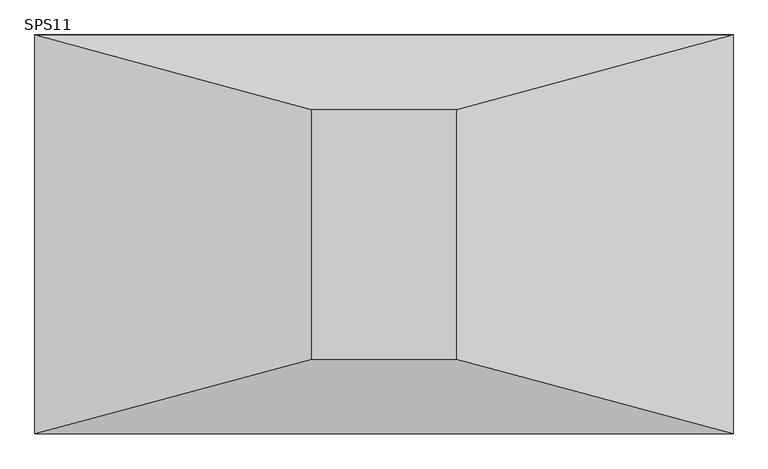
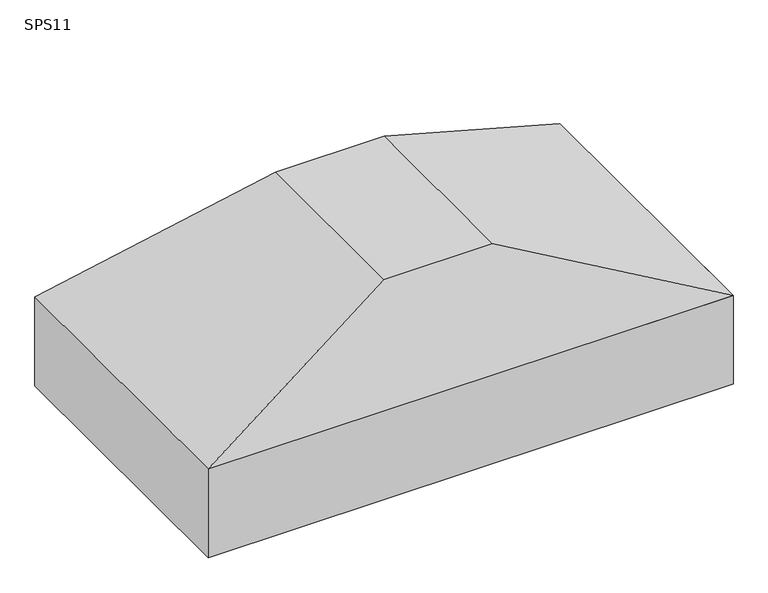
"""IFC4 building model written with IfcOpenShell, lengths in millimetres: fastener geometry, TQS - Sapata : SPS11."""

import ifcopenshell
import ifcopenshell.guid

model = None  # the IFC model being written
_history = None  # IfcOwnerHistory: only IFC2X3 demands one
_inside = {}  # id of a spatial element -> (the spatial element, [elements in it])
_under = {}  # id of a project, library or spatial element -> (it, [spatial elements below it])
_declared = {}  # id of a project -> (the project, [libraries it declares])
_typed = {}  # id of a type object -> (the type object, [elements of that type])
_made_of = {}  # id of a material, layer set ... -> (it, [elements and type objects made of it])


def new_model(schema):
    """Start an empty IFC model of exactly this schema.

    Asked for "IFC4X3", IfcOpenShell would pick the latest addendum, in which some entities
    have other attributes; the version numbers below select the first issue.
    IFC2X3 requires an IfcOwnerHistory on every rooted entity: one is made here for all.
    """
    global model, _history
    if schema == "IFC4X3":
        model = ifcopenshell.file(schema_version=(4, 3, 0, 0))
    else:
        model = ifcopenshell.file(schema=schema)
    _inside.clear()
    _under.clear()
    _declared.clear()
    _typed.clear()
    _made_of.clear()
    _history = None
    if model.schema == "IFC2X3":
        org = make("IfcOrganization", Name="unknown")
        user = make(
            "IfcPersonAndOrganization",
            ThePerson=make("IfcPerson", FamilyName="unknown"),
            TheOrganization=org,
        )
        app = make(
            "IfcApplication",
            ApplicationDeveloper=org,
            Version="unknown",
            ApplicationFullName="unknown",
            ApplicationIdentifier="unknown",
        )
        _history = make(
            "IfcOwnerHistory",
            OwningUser=user,
            OwningApplication=app,
            ChangeAction="ADDED",
            CreationDate=0,
        )
    return model


def make(cls, **values):
    """One entity of the class cls with the attributes given. An attribute that is None is left unset."""
    return model.create_entity(
        cls, **{name: value for name, value in values.items() if value is not None}
    )


def rooted(cls, **values):
    """An entity with a GlobalId (a new one), such as an element, a storey or a relation."""
    return make(cls, GlobalId=ifcopenshell.guid.new(), OwnerHistory=_history, **values)


def si_unit(unit_type, name, prefix=None):
    """IfcSIUnit, for example si_unit("LENGTHUNIT", "METRE", prefix="MILLI")."""
    return make("IfcSIUnit", UnitType=unit_type, Prefix=prefix, Name=name)


def assignment(units):
    """IfcUnitAssignment: the units of a project."""
    return None if units is None else make("IfcUnitAssignment", Units=units)


def point(xyz):
    """IfcCartesianPoint."""
    return None if xyz is None else make("IfcCartesianPoint", Coordinates=xyz)


def direction(xyz):
    """IfcDirection."""
    return None if xyz is None else make("IfcDirection", DirectionRatios=xyz)


def frame(location, z_axis=None, x_axis=None):
    """IfcAxis2Placement3D, a coordinate frame: its origin and axes. An axis left out is left unset."""
    return make(
        "IfcAxis2Placement3D",
        Location=point(location),
        Axis=direction(z_axis),
        RefDirection=direction(x_axis),
    )


def origin():
    """The frame at (0, 0, 0) with its axes left unset."""
    return frame((0.0, 0.0, 0.0))


def place(relative_to, where):
    """IfcLocalPlacement: puts the frame where relative to a parent placement (None: the world)."""
    return make(
        "IfcLocalPlacement", PlacementRelTo=relative_to, RelativePlacement=where
    )


def context(
    kind, dimensions, precision=None, world=None, true_north=None, identifier=None
):
    """IfcGeometricRepresentationContext, for example the 3D "Model" context."""
    return make(
        "IfcGeometricRepresentationContext",
        ContextIdentifier=identifier,
        ContextType=kind,
        CoordinateSpaceDimension=dimensions,
        Precision=precision,
        WorldCoordinateSystem=world,
        TrueNorth=true_north,
    )


def project(units=None, contexts=None):
    """IfcProject with its units and contexts."""
    return rooted(
        "IfcProject",
        Name="project",
        RepresentationContexts=contexts,
        UnitsInContext=assignment(units),
    )


def spatial(cls, under=None, at=None, **own):
    """A site, building, storey or space (cls), placed at a placement, below another one or the project."""
    s = rooted(cls, ObjectPlacement=at, **own)
    if under is not None:
        _under.setdefault(under.id(), (under, []))[1].append(s)
    return s


def polyline(points):
    """IfcPolyline through the points."""
    return make("IfcPolyline", Points=[point(p) for p in points])


def outline(outer, holes=None, kind="AREA"):
    """IfcArbitraryClosedProfileDef: a profile drawn as a closed curve; with holes, ...WithVoids."""
    if holes is None:
        return make("IfcArbitraryClosedProfileDef", ProfileType=kind, OuterCurve=outer)
    return make(
        "IfcArbitraryProfileDefWithVoids",
        ProfileType=kind,
        OuterCurve=outer,
        InnerCurves=holes,
    )


def extrude(swept, where, along, depth):
    """IfcExtrudedAreaSolid: the profile swept, set in the frame where, extruded along a direction by depth."""
    return make(
        "IfcExtrudedAreaSolid",
        SweptArea=swept,
        Position=where,
        ExtrudedDirection=direction(along),
        Depth=depth,
    )


def faces_of(points, faces, orient=None, outer=None):
    """IfcFace entities. A face is a list of loops; a loop is a list of indices into points, from 0.

    orient and outer hold one flag for each loop. By default every Orientation is true, the
    first loop of a face is its IfcFaceOuterBound and the others are IfcFaceBound.
    """
    made = []
    for i, loops in enumerate(faces):
        bounds = []
        for j, loop in enumerate(loops):
            is_outer = j == 0 if outer is None else outer[i][j]
            bounds.append(
                make(
                    "IfcFaceOuterBound" if is_outer else "IfcFaceBound",
                    Bound=make("IfcPolyLoop", Polygon=[points[k] for k in loop]),
                    Orientation=True if orient is None else orient[i][j],
                )
            )
        made.append(make("IfcFace", Bounds=bounds))
    return made


def faceted_brep(points, faces, orient=None, outer=None, voids=None):
    """IfcFacetedBrep: a solid bounded by flat faces; with voids (closed shells), ...WithVoids."""
    shared = [point(p) for p in points]
    hull = make("IfcClosedShell", CfsFaces=faces_of(shared, faces, orient, outer))
    if voids is None:
        return make("IfcFacetedBrep", Outer=hull)
    return make(
        "IfcFacetedBrepWithVoids",
        Outer=hull,
        Voids=[
            make(cls, CfsFaces=faces_of(shared, fs, o, b)) for cls, fs, o, b in voids
        ],
    )


def shape(context_of_items, identifier, shape_type, items):
    """IfcShapeRepresentation: the items that make up one representation, for example the "Body"."""
    return make(
        "IfcShapeRepresentation",
        ContextOfItems=context_of_items,
        RepresentationIdentifier=identifier,
        RepresentationType=shape_type,
        Items=items,
    )


def source(mapping_origin, context_of_items, identifier, shape_type, items):
    """IfcRepresentationMap: a shape defined once, which mapped items show again and again."""
    return make(
        "IfcRepresentationMap",
        MappingOrigin=mapping_origin,
        MappedRepresentation=shape(context_of_items, identifier, shape_type, items),
    )


def transform(
    local_origin,
    x_axis=None,
    y_axis=None,
    z_axis=None,
    scale=None,
    scale2=None,
    scale3=None,
    uniform=True,
):
    """IfcCartesianTransformationOperator3D, or its non-uniform kind. x_axis, y_axis, z_axis: its Axis1, 2, 3."""
    if uniform:
        return make(
            "IfcCartesianTransformationOperator3D",
            Axis1=direction(x_axis),
            Axis2=direction(y_axis),
            LocalOrigin=point(local_origin),
            Scale=scale,
            Axis3=direction(z_axis),
        )
    return make(
        "IfcCartesianTransformationOperator3DnonUniform",
        Axis1=direction(x_axis),
        Axis2=direction(y_axis),
        LocalOrigin=point(local_origin),
        Scale=scale,
        Axis3=direction(z_axis),
        Scale2=scale2,
        Scale3=scale3,
    )


def mapped(mapping_source, mapping_target):
    """IfcMappedItem: shows the shape of a source again, moved by a transform."""
    return make(
        "IfcMappedItem", MappingSource=mapping_source, MappingTarget=mapping_target
    )


def made_of(thing, what):
    """Note that an element or type object is made of a material, layer set ...; save() writes the relation."""
    if what is not None:
        _made_of.setdefault(what.id(), (what, []))[1].append(thing)
    return thing


def element(
    cls,
    number,
    at=None,
    inside=None,
    cuts=None,
    type_object=None,
    material=None,
    context=None,
    identifier="Body",
    shape_type=None,
    held_by="IfcProductDefinitionShape",
    body=None,
    shapes=None,
    **own,
):
    """One element of the class cls, such as IfcWall. Its Tag is "e" and its number.

    at: its placement. inside: the storey or other place that contains it. cuts: it is an
    opening in that element (IfcRelVoidsElement). A single representation is given by context,
    identifier, shape_type and body (its items); several are given by shapes. held_by: the class
    of the entity that holds the representations. save() writes the other relations.
    """
    e = rooted(cls, Tag="e%d" % number, ObjectPlacement=at, **own)
    if body is not None:
        shapes = [shape(context, identifier, shape_type, body)]
    if shapes is not None:
        e.Representation = make(held_by, Representations=shapes)
    if inside is not None:
        _inside.setdefault(inside.id(), (inside, []))[1].append(e)
    if cuts is not None:
        rooted(
            "IfcRelVoidsElement", RelatingBuildingElement=cuts, RelatedOpeningElement=e
        )
    if type_object is not None:
        _typed.setdefault(type_object.id(), (type_object, []))[1].append(e)
    return made_of(e, material)


def aggregate(whole, parts):
    """IfcRelAggregates: a whole, such as a stair, and the parts it consists of."""
    return rooted("IfcRelAggregates", RelatingObject=whole, RelatedObjects=parts)


def save(model, path):
    """Write the relations noted so far, then the file.

    IfcRelAggregates (storeys below a building ...), IfcRelContainedInSpatialStructure (elements
    in a storey), IfcRelDefinesByType, IfcRelAssociatesMaterial and IfcRelDeclares: one each for
    every whole, place, type object, material and project.
    """
    for whole, parts in _under.values():
        aggregate(whole, parts)
    for where, things in _inside.values():
        rooted(
            "IfcRelContainedInSpatialStructure",
            RelatedElements=things,
            RelatingStructure=where,
        )
    for kind, things in _typed.values():
        rooted("IfcRelDefinesByType", RelatedObjects=things, RelatingType=kind)
    for what, things in _made_of.values():
        rooted("IfcRelAssociatesMaterial", RelatedObjects=things, RelatingMaterial=what)
    for by, libraries in _declared.values():
        rooted("IfcRelDeclares", RelatingContext=by, RelatedDefinitions=libraries)
    model.write(path)


def sps11_3ae28187(model_context):
    return source(origin(), model_context, "Body", "SolidModel", [
        faceted_brep([(-55.0, 50.0, 0.0), (-345.0, 50.0, 0.0), (-345.0, -450.0, 0.0), (-55.0, -450.0, 0.0), (500.0, 200.0, -250.0), (500.0, -600.0, -250.0), (-900.0, -600.0, -250.0), (-900.0, 200.0, -250.0)], [[[0, 1, 2, 3]], [[4, 5, 6, 7]], [[4, 7, 1, 0]], [[7, 6, 2, 1]], [[6, 5, 3, 2]], [[5, 4, 0, 3]]]),
        extrude(outline(polyline([(500.0, 200.0), (500.0, -600.0), (-900.0, -600.0), (-900.0, 200.0), (500.0, 200.0)])), frame((0.0, 0.0, -500.0), z_axis=(0.0, 0.0, 1.0), x_axis=(1.0, 0.0, 0.0)), (0.0, 0.0, 1.0), 250.0),
    ])


if __name__ == "__main__":
    model = new_model("IFC4")
    model_context = context("Model", 3, world=origin())
    ifc_project = project(units=[si_unit("LENGTHUNIT", "METRE", prefix="MILLI")], contexts=[model_context])
    site = spatial("IfcSite", under=ifc_project)
    building = spatial("IfcBuilding", under=site)
    placement = place(None, origin())
    sps11_shape = sps11_3ae28187(model_context)
    element("IfcFastener", 1, ObjectType="TQS - Sapata : SPS11", at=placement, inside=building, context=model_context, shape_type="MappedRepresentation", body=[
        mapped(sps11_shape, transform((0.0, 0.0, 0.0), x_axis=(1.0, 0.0, 0.0), y_axis=(0.0, 1.0, 0.0), z_axis=(0.0, 0.0, 1.0))),
    ])
    save(model, "model.ifc")

# Revit data of these elements
# Type "TQS - Sapata : SPS11"
#   TY = 0.50 m
#   TX = 0.29 m
#   HS = 0.50 m
#   H0 = 0.25 m
#   EXCYABS = 0.40 m
#   EXCY = 0.00 m
#   EXCXABS = 0.70 m
#   EXCX = 0.00 m
#   DIMY = 0.80 m
#   DIMX = 1.40 m
#   Material estrutural = Concreto - Concreto concretado no local
#   Width = 0
#   Length = 0
# Element 1 (IfcFastener, "TQS - Sapata : SPS11")
#   Materials on its faces: "Concreto - Concreto concretado no local"
# Materials
#   "Concreto - Concreto concretado no local": class "Concreto", colour RGB 192 192 192, transparency 0
